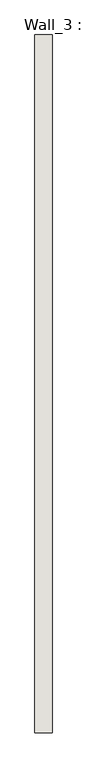
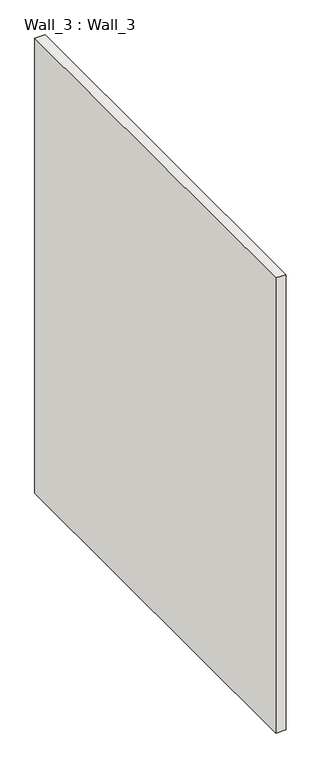
"""IFC4 building model written with IfcOpenShell, lengths in millimetres: wall geometry, Wall_3 : Wall_3."""

from ifc_helpers import new_model, si_unit, origin, origin_with_axes, place, context, project, spatial, polyline, outline, extrude, source, transform, mapped, element, save


def wall_3_wall_3_2bae312e(model_context):
    return source(origin(), model_context, "Body", "SweptSolid", [
        extrude(outline(polyline([(100.0, 11970.0), (100.0, 7890.0), (0.0, 7890.0), (0.0, 11970.0), (100.0, 11970.0)])), origin_with_axes(), (0.0, 0.0, 1.0), 4700.0),
    ])


if __name__ == "__main__":
    model = new_model("IFC4")
    model_context = context("Model", 3, world=origin())
    ifc_project = project(units=[si_unit("LENGTHUNIT", "METRE", prefix="MILLI")], contexts=[model_context])
    site = spatial("IfcSite", under=ifc_project)
    building = spatial("IfcBuilding", under=site)
    placement = place(None, origin())
    wall_3_wall_3_shape = wall_3_wall_3_2bae312e(model_context)
    element("IfcWall", 1, ObjectType="Wall_3 : Wall_3", at=placement, inside=building, context=model_context, shape_type="MappedRepresentation", body=[
        mapped(wall_3_wall_3_shape, transform((0.0, 0.0, 0.0), x_axis=(1.0, 0.0, 0.0), y_axis=(0.0, 1.0, 0.0), z_axis=(0.0, 0.0, 1.0))),
    ])
    save(model, "model.ifc")

# Revit data of these elements
# Type "Wall_3 : Wall_3"
#   NameOverride = "Wall_3"
# Element 1 (IfcWall, "Wall_3 : Wall_3")
#   Materials on its faces: "IfcSurfaceStyle #33"
# Materials
#   "IfcSurfaceStyle #33": class "Unassigned", colour RGB 214 214 214, transparency 0
